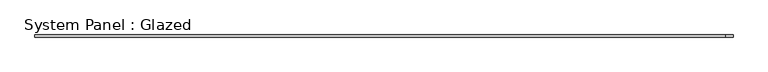
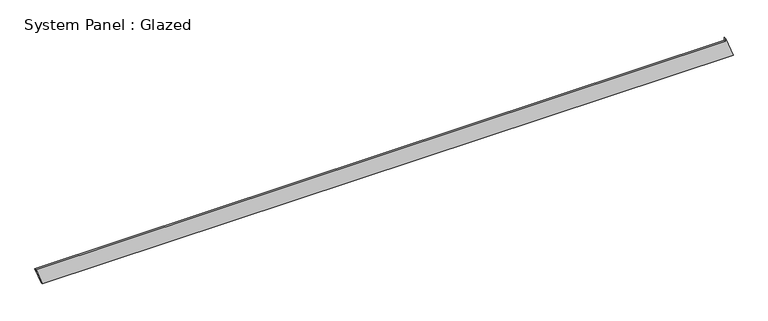
"""IFC4 building model written with IfcOpenShell, lengths in millimetres: plate geometry, System Panel : Glazed."""

from ifc_helpers import new_model, si_unit, frame, origin, place, context, project, spatial, polyline, outline, extrude, source, transform, mapped, element, save


def system_panel_glazed_d7fe694e(model_context):
    return source(origin(), model_context, "Body", "SweptSolid", [
        extrude(outline(polyline([(0.0, -3964.2777152), (0.0, 4035.2773263), (233.2527248, 3950.1929605), (197.8973858, 3950.1906717), (198.4143393, -4035.2773263), (0.0, -3964.2777152)])), frame((0.0, -49.5, 0.0), z_axis=(0.0, 1.0, 0.0), x_axis=(0.0, 0.0, 1.0)), (0.0, 0.0, 1.0), 25.0),
    ])


if __name__ == "__main__":
    model = new_model("IFC4")
    model_context = context("Model", 3, world=origin())
    ifc_project = project(units=[si_unit("LENGTHUNIT", "METRE", prefix="MILLI")], contexts=[model_context])
    site = spatial("IfcSite", under=ifc_project)
    building = spatial("IfcBuilding", under=site)
    placement = place(None, origin())
    system_panel_glazed_shape = system_panel_glazed_d7fe694e(model_context)
    element("IfcPlate", 1, ObjectType="System Panel : Glazed", at=placement, inside=building, context=model_context, shape_type="MappedRepresentation", body=[
        mapped(system_panel_glazed_shape, transform((0.0, 0.0, 0.0), x_axis=(1.0, 0.0, 0.0), y_axis=(0.0, 1.0, 0.0), z_axis=(0.0, 0.0, 1.0))),
    ])
    save(model, "model.ifc")

# Revit data of these elements
# Element 1 (IfcPlate, "System Panel : Glazed")
#   Materials on its faces: "Glass"
# Materials
#   "Glass": class "Glass", colour RGB 218 227 224, transparency 0.85, Description = "Soda Lime Glass", Cost = 0
